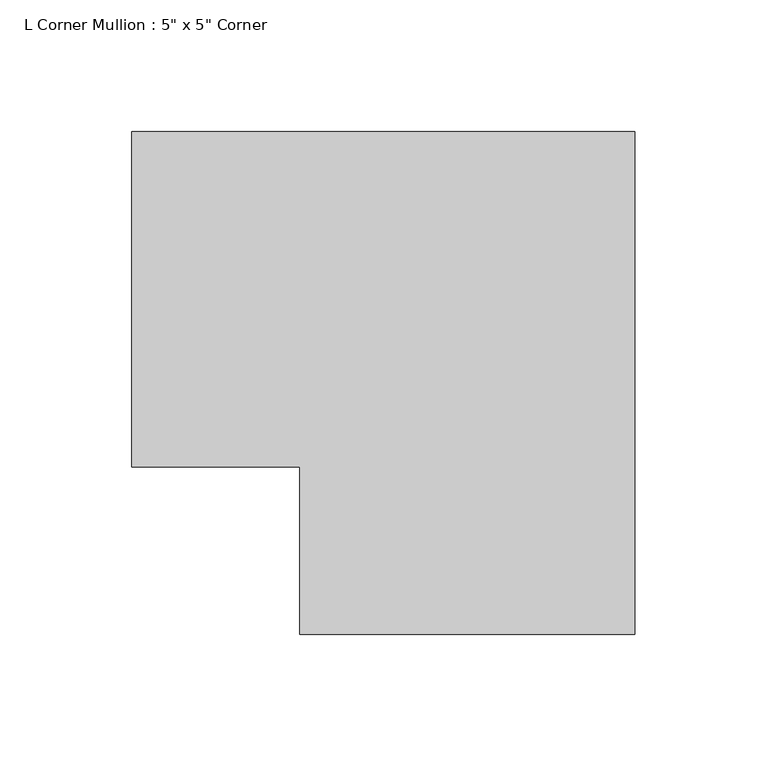
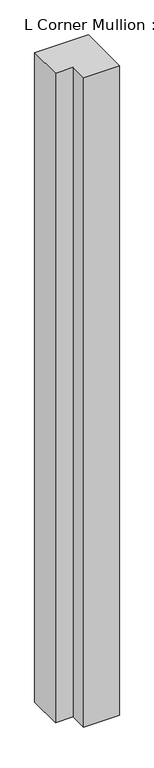
"""IFC4 building model written with IfcOpenShell, lengths in millimetres: member geometry."""

import ifcopenshell
import ifcopenshell.guid

model = None  # the IFC model being written
_history = None  # IfcOwnerHistory: only IFC2X3 demands one
_inside = {}  # id of a spatial element -> (the spatial element, [elements in it])
_under = {}  # id of a project, library or spatial element -> (it, [spatial elements below it])
_declared = {}  # id of a project -> (the project, [libraries it declares])
_typed = {}  # id of a type object -> (the type object, [elements of that type])
_made_of = {}  # id of a material, layer set ... -> (it, [elements and type objects made of it])


def new_model(schema):
    """Start an empty IFC model of exactly this schema.

    Asked for "IFC4X3", IfcOpenShell would pick the latest addendum, in which some entities
    have other attributes; the version numbers below select the first issue.
    IFC2X3 requires an IfcOwnerHistory on every rooted entity: one is made here for all.
    """
    global model, _history
    if schema == "IFC4X3":
        model = ifcopenshell.file(schema_version=(4, 3, 0, 0))
    else:
        model = ifcopenshell.file(schema=schema)
    _inside.clear()
    _under.clear()
    _declared.clear()
    _typed.clear()
    _made_of.clear()
    _history = None
    if model.schema == "IFC2X3":
        org = make("IfcOrganization", Name="unknown")
        user = make(
            "IfcPersonAndOrganization",
            ThePerson=make("IfcPerson", FamilyName="unknown"),
            TheOrganization=org,
        )
        app = make(
            "IfcApplication",
            ApplicationDeveloper=org,
            Version="unknown",
            ApplicationFullName="unknown",
            ApplicationIdentifier="unknown",
        )
        _history = make(
            "IfcOwnerHistory",
            OwningUser=user,
            OwningApplication=app,
            ChangeAction="ADDED",
            CreationDate=0,
        )
    return model


def make(cls, **values):
    """One entity of the class cls with the attributes given. An attribute that is None is left unset."""
    return model.create_entity(
        cls, **{name: value for name, value in values.items() if value is not None}
    )


def rooted(cls, **values):
    """An entity with a GlobalId (a new one), such as an element, a storey or a relation."""
    return make(cls, GlobalId=ifcopenshell.guid.new(), OwnerHistory=_history, **values)


def si_unit(unit_type, name, prefix=None):
    """IfcSIUnit, for example si_unit("LENGTHUNIT", "METRE", prefix="MILLI")."""
    return make("IfcSIUnit", UnitType=unit_type, Prefix=prefix, Name=name)


def assignment(units):
    """IfcUnitAssignment: the units of a project."""
    return None if units is None else make("IfcUnitAssignment", Units=units)


def point(xyz):
    """IfcCartesianPoint."""
    return None if xyz is None else make("IfcCartesianPoint", Coordinates=xyz)


def direction(xyz):
    """IfcDirection."""
    return None if xyz is None else make("IfcDirection", DirectionRatios=xyz)


def frame(location, z_axis=None, x_axis=None):
    """IfcAxis2Placement3D, a coordinate frame: its origin and axes. An axis left out is left unset."""
    return make(
        "IfcAxis2Placement3D",
        Location=point(location),
        Axis=direction(z_axis),
        RefDirection=direction(x_axis),
    )


def origin():
    """The frame at (0, 0, 0) with its axes left unset."""
    return frame((0.0, 0.0, 0.0))


def place(relative_to, where):
    """IfcLocalPlacement: puts the frame where relative to a parent placement (None: the world)."""
    return make(
        "IfcLocalPlacement", PlacementRelTo=relative_to, RelativePlacement=where
    )


def context(
    kind, dimensions, precision=None, world=None, true_north=None, identifier=None
):
    """IfcGeometricRepresentationContext, for example the 3D "Model" context."""
    return make(
        "IfcGeometricRepresentationContext",
        ContextIdentifier=identifier,
        ContextType=kind,
        CoordinateSpaceDimension=dimensions,
        Precision=precision,
        WorldCoordinateSystem=world,
        TrueNorth=true_north,
    )


def project(units=None, contexts=None):
    """IfcProject with its units and contexts."""
    return rooted(
        "IfcProject",
        Name="project",
        RepresentationContexts=contexts,
        UnitsInContext=assignment(units),
    )


def spatial(cls, under=None, at=None, **own):
    """A site, building, storey or space (cls), placed at a placement, below another one or the project."""
    s = rooted(cls, ObjectPlacement=at, **own)
    if under is not None:
        _under.setdefault(under.id(), (under, []))[1].append(s)
    return s


def polyline(points):
    """IfcPolyline through the points."""
    return make("IfcPolyline", Points=[point(p) for p in points])


def outline(outer, holes=None, kind="AREA"):
    """IfcArbitraryClosedProfileDef: a profile drawn as a closed curve; with holes, ...WithVoids."""
    if holes is None:
        return make("IfcArbitraryClosedProfileDef", ProfileType=kind, OuterCurve=outer)
    return make(
        "IfcArbitraryProfileDefWithVoids",
        ProfileType=kind,
        OuterCurve=outer,
        InnerCurves=holes,
    )


def extrude(swept, where, along, depth):
    """IfcExtrudedAreaSolid: the profile swept, set in the frame where, extruded along a direction by depth."""
    return make(
        "IfcExtrudedAreaSolid",
        SweptArea=swept,
        Position=where,
        ExtrudedDirection=direction(along),
        Depth=depth,
    )


def shape(context_of_items, identifier, shape_type, items):
    """IfcShapeRepresentation: the items that make up one representation, for example the "Body"."""
    return make(
        "IfcShapeRepresentation",
        ContextOfItems=context_of_items,
        RepresentationIdentifier=identifier,
        RepresentationType=shape_type,
        Items=items,
    )


def source(mapping_origin, context_of_items, identifier, shape_type, items):
    """IfcRepresentationMap: a shape defined once, which mapped items show again and again."""
    return make(
        "IfcRepresentationMap",
        MappingOrigin=mapping_origin,
        MappedRepresentation=shape(context_of_items, identifier, shape_type, items),
    )


def transform(
    local_origin,
    x_axis=None,
    y_axis=None,
    z_axis=None,
    scale=None,
    scale2=None,
    scale3=None,
    uniform=True,
):
    """IfcCartesianTransformationOperator3D, or its non-uniform kind. x_axis, y_axis, z_axis: its Axis1, 2, 3."""
    if uniform:
        return make(
            "IfcCartesianTransformationOperator3D",
            Axis1=direction(x_axis),
            Axis2=direction(y_axis),
            LocalOrigin=point(local_origin),
            Scale=scale,
            Axis3=direction(z_axis),
        )
    return make(
        "IfcCartesianTransformationOperator3DnonUniform",
        Axis1=direction(x_axis),
        Axis2=direction(y_axis),
        LocalOrigin=point(local_origin),
        Scale=scale,
        Axis3=direction(z_axis),
        Scale2=scale2,
        Scale3=scale3,
    )


def mapped(mapping_source, mapping_target):
    """IfcMappedItem: shows the shape of a source again, moved by a transform."""
    return make(
        "IfcMappedItem", MappingSource=mapping_source, MappingTarget=mapping_target
    )


def made_of(thing, what):
    """Note that an element or type object is made of a material, layer set ...; save() writes the relation."""
    if what is not None:
        _made_of.setdefault(what.id(), (what, []))[1].append(thing)
    return thing


def element(
    cls,
    number,
    at=None,
    inside=None,
    cuts=None,
    type_object=None,
    material=None,
    context=None,
    identifier="Body",
    shape_type=None,
    held_by="IfcProductDefinitionShape",
    body=None,
    shapes=None,
    **own,
):
    """One element of the class cls, such as IfcWall. Its Tag is "e" and its number.

    at: its placement. inside: the storey or other place that contains it. cuts: it is an
    opening in that element (IfcRelVoidsElement). A single representation is given by context,
    identifier, shape_type and body (its items); several are given by shapes. held_by: the class
    of the entity that holds the representations. save() writes the other relations.
    """
    e = rooted(cls, Tag="e%d" % number, ObjectPlacement=at, **own)
    if body is not None:
        shapes = [shape(context, identifier, shape_type, body)]
    if shapes is not None:
        e.Representation = make(held_by, Representations=shapes)
    if inside is not None:
        _inside.setdefault(inside.id(), (inside, []))[1].append(e)
    if cuts is not None:
        rooted(
            "IfcRelVoidsElement", RelatingBuildingElement=cuts, RelatedOpeningElement=e
        )
    if type_object is not None:
        _typed.setdefault(type_object.id(), (type_object, []))[1].append(e)
    return made_of(e, material)


def aggregate(whole, parts):
    """IfcRelAggregates: a whole, such as a stair, and the parts it consists of."""
    return rooted("IfcRelAggregates", RelatingObject=whole, RelatedObjects=parts)


def save(model, path):
    """Write the relations noted so far, then the file.

    IfcRelAggregates (storeys below a building ...), IfcRelContainedInSpatialStructure (elements
    in a storey), IfcRelDefinesByType, IfcRelAssociatesMaterial and IfcRelDeclares: one each for
    every whole, place, type object, material and project.
    """
    for whole, parts in _under.values():
        aggregate(whole, parts)
    for where, things in _inside.values():
        rooted(
            "IfcRelContainedInSpatialStructure",
            RelatedElements=things,
            RelatingStructure=where,
        )
    for kind, things in _typed.values():
        rooted("IfcRelDefinesByType", RelatedObjects=things, RelatingType=kind)
    for what, things in _made_of.values():
        rooted("IfcRelAssociatesMaterial", RelatedObjects=things, RelatingMaterial=what)
    for by, libraries in _declared.values():
        rooted("IfcRelDeclares", RelatingContext=by, RelatedDefinitions=libraries)
    model.write(path)


def member_47e31e63(model_context):
    return source(origin(), model_context, "Body", "SweptSolid", [
        extrude(outline(polyline([(-63.5, -127.0), (-63.5, -63.5), (-127.0, -63.5), (-127.0, 63.5), (63.5, 63.5), (63.5, -127.0), (-63.5, -127.0)])), frame((0.0, 0.0, -2438.4), z_axis=(0.0, 0.0, 1.0), x_axis=(1.0, 0.0, 0.0)), (0.0, 0.0, 1.0), 2438.4),
    ])


if __name__ == "__main__":
    model = new_model("IFC4")
    model_context = context("Model", 3, world=origin())
    ifc_project = project(units=[si_unit("LENGTHUNIT", "METRE", prefix="MILLI")], contexts=[model_context])
    site = spatial("IfcSite", under=ifc_project)
    building = spatial("IfcBuilding", under=site)
    placement = place(None, origin())
    member_shape = member_47e31e63(model_context)
    element("IfcMember", 1, ObjectType="L Corner Mullion : 5\" x 5\" Corner", at=placement, inside=building, context=model_context, shape_type="MappedRepresentation", body=[
        mapped(member_shape, transform((0.0, 0.0, 0.0), x_axis=(1.0, 0.0, 0.0), y_axis=(0.0, 1.0, 0.0), z_axis=(0.0, 0.0, 1.0))),
    ])
    save(model, "model.ifc")

# Revit data of these elements
# Type "L Corner Mullion : 5\" x 5\" Corner"
#   built-in parameter 1007355 = 0.416667 (stored number, unit not read)
#   built-in parameter 1007354 = 0.416667 (stored number, unit not read)
#   built-in parameter 1007304 = 0.416667 (stored number, unit not read)
# Element 1 (IfcMember, "L Corner Mullion : 5\" x 5\" Corner")
#   Materials on its faces: "Metal - Aluminum, Black-Annodized"
# Materials
#   "Metal - Aluminum, Black-Annodized": class "Metal", colour RGB 10 10 10, transparency 0, Cost = 0
